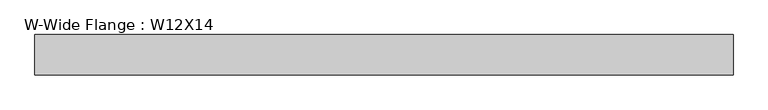
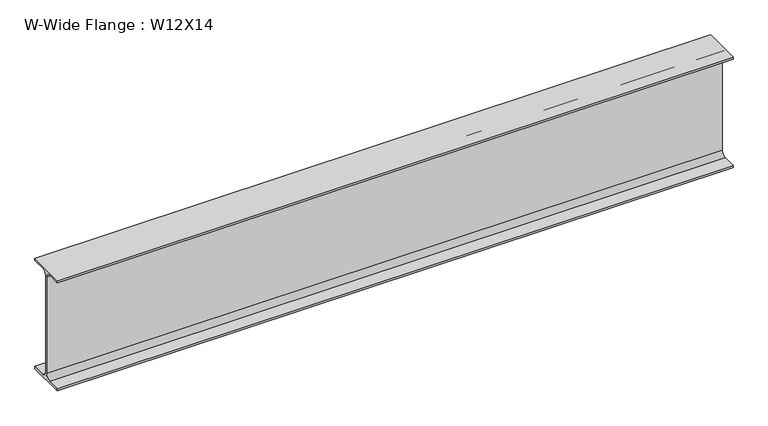
"""IFC4 building model written with IfcOpenShell, lengths in millimetres: beam geometry, W-Wide Flange : W12X14."""

from ifc_helpers import new_model, si_unit, point, frame, frame_2d, origin, place, context, project, spatial, polyline, circle_curve, trimmed, segment, composite_curve, outline, extrude, source, transform, mapped, element, save


def w_wide_flange_w12x14_ef09f6af(model_context):
    return source(origin(), model_context, "Body", "SweptSolid", [
        extrude(outline(composite_curve([segment(polyline([(50.419, -145.415), (50.419, -151.13), (-50.419, -151.13), (-50.419, -145.415), (-15.875, -145.415)]), True, "CONTINUOUS"), segment(trimmed(circle_curve(frame_2d((-15.875, -132.08)), 13.335), [point((-15.875, -145.415))], [point((-2.54, -132.08))], True, "CARTESIAN"), True, "CONTINUOUS"), segment(polyline([(-2.54, -132.08), (-2.54, 132.08)]), True, "CONTINUOUS"), segment(trimmed(circle_curve(frame_2d((-15.875, 132.08)), 13.335), [point((-2.54, 132.08))], [point((-15.875, 145.415))], True, "CARTESIAN"), True, "CONTINUOUS"), segment(polyline([(-15.875, 145.415), (-50.419, 145.415), (-50.419, 151.13), (50.419, 151.13), (50.419, 145.415), (15.875, 145.415)]), True, "CONTINUOUS"), segment(trimmed(circle_curve(frame_2d((15.875, 132.08)), 13.335), [point((15.875, 145.415))], [point((2.54, 132.08))], True, "CARTESIAN"), True, "CONTINUOUS"), segment(polyline([(2.54, 132.08), (2.54, -132.08)]), True, "CONTINUOUS"), segment(trimmed(circle_curve(frame_2d((15.875, -132.08)), 13.335), [point((2.54, -132.08))], [point((15.875, -145.415))], True, "CARTESIAN"), True, "CONTINUOUS"), segment(polyline([(15.875, -145.415), (50.419, -145.415)]), True, "CONTINUOUS")], self_intersect=False)), frame((-875.6649994, 0.0, 0.0), z_axis=(1.0, 0.0, 0.0), x_axis=(0.0, 1.0, 0.0)), (0.0, 0.0, 1.0), 1750.0599994),
    ])


if __name__ == "__main__":
    model = new_model("IFC4")
    model_context = context("Model", 3, world=origin())
    ifc_project = project(units=[si_unit("LENGTHUNIT", "METRE", prefix="MILLI")], contexts=[model_context])
    site = spatial("IfcSite", under=ifc_project)
    building = spatial("IfcBuilding", under=site)
    placement = place(None, origin())
    w_wide_flange_w12x14_shape = w_wide_flange_w12x14_ef09f6af(model_context)
    element("IfcBeam", 1, ObjectType="W-Wide Flange : W12X14", at=placement, inside=building, context=model_context, shape_type="MappedRepresentation", body=[
        mapped(w_wide_flange_w12x14_shape, transform((0.0, 0.0, 0.0), x_axis=(1.0, 0.0, 0.0), y_axis=(0.0, 1.0, 0.0), z_axis=(0.0, 0.0, 1.0))),
    ])
    save(model, "model.ifc")

# Revit data of these elements
# Type "W-Wide Flange : W12X14"
#   Assembly Code = "B10"
#   W = 14
#   Length [instance default] = 5' - 0"
#   bf = 0' - 3.97"
#   d = 0' - 11.9"
#   k = 0' - 0 3/4"
#   k2 = 0' - 0.525"
#   tf = 0' - 0.225"
#   tw = 0' - 0.2"
#   A = 0.0288889 SF
#   Structural Material [instance default] = Steel ASTM A992
# Element 1 (IfcBeam, "W-Wide Flange : W12X14")
#   Materials on its faces: "Steel ASTM A992"
# Materials
#   "Steel ASTM A992": class "Metal", colour RGB 199 199 199, transparency 0, Description = "Structural steel 50ksi", Cost = 0
